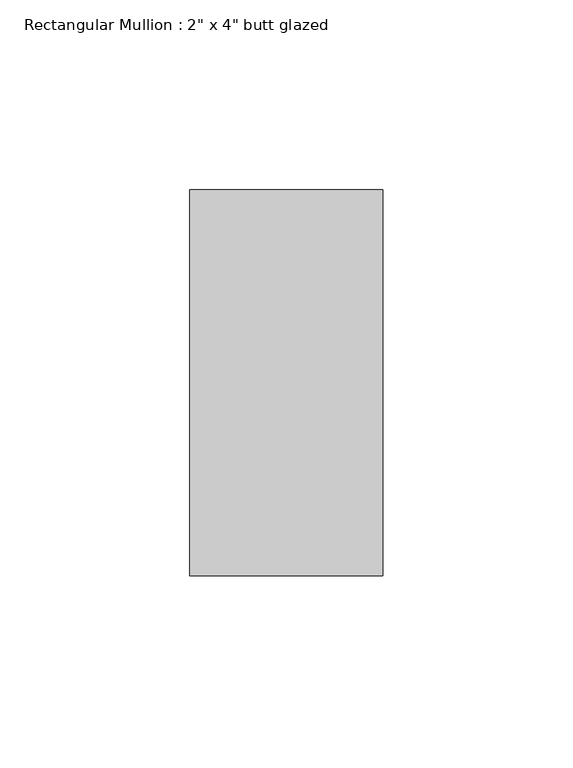
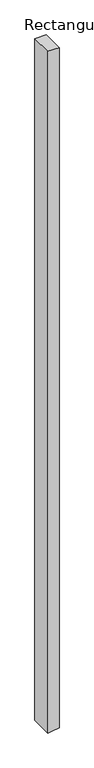
"""IFC4 building model written with IfcOpenShell, lengths in millimetres: member geometry."""

from ifc_helpers import new_model, si_unit, frame, origin, place, context, project, spatial, polyline, outline, extrude, source, transform, mapped, element, save


def member_363eeca2(model_context):
    return source(origin(), model_context, "Body", "SweptSolid", [
        extrude(outline(polyline([(0.0, 25.4), (0.0, -25.4), (-3265.9198776, -25.4), (-3263.0555363, -8.4783527), (-3257.3209193, 25.4), (0.0, 25.4)])), frame((0.0, -114.3, 0.0), z_axis=(0.0, 1.0, 0.0), x_axis=(0.0, 0.0, 1.0)), (0.0, 0.0, 1.0), 101.6),
    ])


if __name__ == "__main__":
    model = new_model("IFC4")
    model_context = context("Model", 3, world=origin())
    ifc_project = project(units=[si_unit("LENGTHUNIT", "METRE", prefix="MILLI")], contexts=[model_context])
    site = spatial("IfcSite", under=ifc_project)
    building = spatial("IfcBuilding", under=site)
    placement = place(None, origin())
    member_shape = member_363eeca2(model_context)
    element("IfcMember", 1, ObjectType="Rectangular Mullion : 2\" x 4\" butt glazed", at=placement, inside=building, context=model_context, shape_type="MappedRepresentation", body=[
        mapped(member_shape, transform((0.0, 0.0, 0.0), x_axis=(1.0, 0.0, 0.0), y_axis=(0.0, 1.0, 0.0), z_axis=(0.0, 0.0, 1.0))),
    ])
    save(model, "model.ifc")

# Revit data of these elements
# Type "Rectangular Mullion : 2\" x 4\" butt glazed"
#   built-in parameter 1007351 = -0.208333 (stored number, unit not read)
#   built-in parameter 1007304 = 0.333333 (stored number, unit not read)
#   built-in parameter 1007301 = 0.0833333 (stored number, unit not read)
#   built-in parameter 1007300 = 0.0833333 (stored number, unit not read)
# Element 1 (IfcMember, "Rectangular Mullion : 2\" x 4\" butt glazed")
#   Materials on its faces: "PAINTED STEEL C CHANNEL"
# Materials
#   "PAINTED STEEL C CHANNEL": class "Generic", colour RGB 88 62 61, transparency 0, Cost = 0
